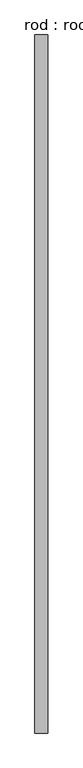
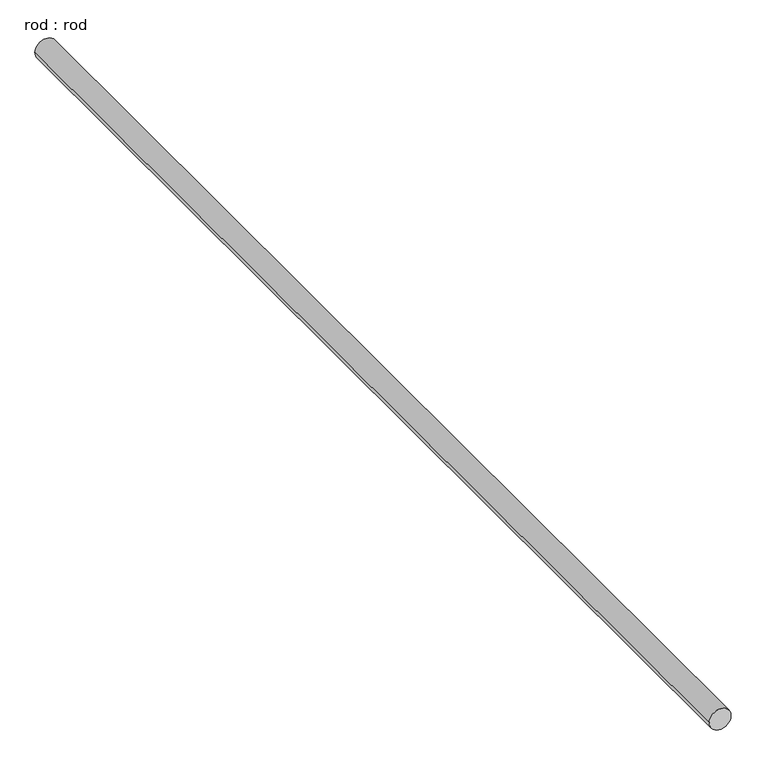
"""IFC4 building model written with IfcOpenShell, lengths in millimetres: proxy geometry, rod : rod."""

from ifc_helpers import new_model, si_unit, point, frame, frame_2d, origin, place, context, project, spatial, circle_curve, trimmed, segment, composite_curve, outline, extrude, source, transform, mapped, element, save


def rod_rod_32cded0c(model_context):
    return source(origin(), model_context, "Body", "SweptSolid", [
        extrude(outline(composite_curve([segment(trimmed(circle_curve(frame_2d((0.0108462, 0.0)), 200.0), [point((0.0108462, 200.0))], [point((0.0108462, -200.0))], False, "CARTESIAN"), True, "CONTINUOUS"), segment(trimmed(circle_curve(frame_2d((0.0108462, 0.0)), 200.0), [point((0.0108462, -200.0))], [point((0.0108462, 200.0))], False, "CARTESIAN"), True, "CONTINUOUS")], self_intersect=False)), frame((0.0, -6629.5622275, 0.0), z_axis=(0.0, 1.0, 0.0), x_axis=(0.0, 0.0, 1.0)), (0.0, 0.0, 1.0), 21444.5816857),
    ])


if __name__ == "__main__":
    model = new_model("IFC4")
    model_context = context("Model", 3, world=origin())
    ifc_project = project(units=[si_unit("LENGTHUNIT", "METRE", prefix="MILLI")], contexts=[model_context])
    site = spatial("IfcSite", under=ifc_project)
    building = spatial("IfcBuilding", under=site)
    placement = place(None, origin())
    rod_rod_shape = rod_rod_32cded0c(model_context)
    element("IfcBuildingElementProxy", 1, Name="rod : rod", ObjectType="rod : rod", at=placement, inside=building, context=model_context, shape_type="MappedRepresentation", body=[
        mapped(rod_rod_shape, transform((0.0, 0.0, 0.0), x_axis=(1.0, 0.0, 0.0), y_axis=(0.0, 1.0, 0.0), z_axis=(0.0, 0.0, 1.0))),
    ])
    save(model, "model.ifc")

# Revit data of these elements
# Type "rod : rod"
#   Default Elevation = 0
